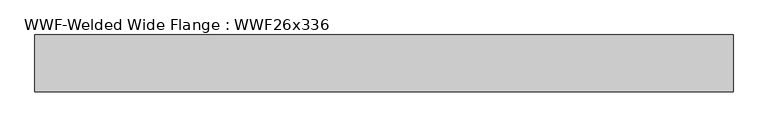
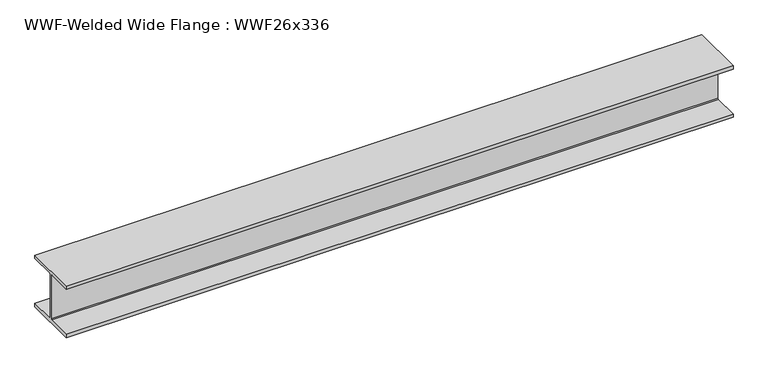
"""IFC4 building model written with IfcOpenShell, lengths in millimetres: beam geometry, WWF-Welded Wide Flange : WWF26x336."""

from ifc_helpers import new_model, si_unit, frame, origin, place, context, project, spatial, polyline, outline, extrude, source, transform, mapped, element, save


def wwf_welded_wide_flange_wwf26x336_71f8c54e(model_context):
    return source(origin(), model_context, "Body", "SweptSolid", [
        extrude(outline(polyline([(324.993, -284.988), (324.993, -324.993), (-324.993, -324.993), (-324.993, -284.988), (-20.6375, -284.988), (-9.9949, -274.3454), (-9.9949, 274.3454), (-20.6375, 284.988), (-324.993, 284.988), (-324.993, 324.993), (324.993, 324.993), (324.993, 284.988), (20.6375, 284.988), (9.9949, 274.3454), (9.9949, -274.3454), (20.6375, -284.988), (324.993, -284.988)])), frame((-3934.8877112, 0.0, 0.0), z_axis=(1.0, 0.0, 0.0), x_axis=(0.0, 1.0, 0.0)), (0.0, 0.0, 1.0), 7999.1183534),
    ])


if __name__ == "__main__":
    model = new_model("IFC4")
    model_context = context("Model", 3, world=origin())
    ifc_project = project(units=[si_unit("LENGTHUNIT", "METRE", prefix="MILLI")], contexts=[model_context])
    site = spatial("IfcSite", under=ifc_project)
    building = spatial("IfcBuilding", under=site)
    placement = place(None, origin())
    wwf_welded_wide_flange_wwf26x336_shape = wwf_welded_wide_flange_wwf26x336_71f8c54e(model_context)
    element("IfcBeam", 1, ObjectType="WWF-Welded Wide Flange : WWF26x336", at=placement, inside=building, context=model_context, shape_type="MappedRepresentation", body=[
        mapped(wwf_welded_wide_flange_wwf26x336_shape, transform((0.0, 0.0, 0.0), x_axis=(1.0, 0.0, 0.0), y_axis=(0.0, 1.0, 0.0), z_axis=(0.0, 0.0, 1.0))),
    ])
    save(model, "model.ifc")

# Revit data of these elements
# Type "WWF-Welded Wide Flange : WWF26x336"
#   Assembly Code = "B10"
#   Nominal d = "12"
#   W = 336
#   Length [instance default] = 1524 mm
#   bf = 649.986 mm
#   d = 649.986 mm
#   k = 20.638 mm
#   tf = 40.005 mm
#   tw = 19.99 mm
#   A = 0.0635483 m²
#   Structural Material [instance default] = Steel ASTM A572
# Element 1 (IfcBeam, "WWF-Welded Wide Flange : WWF26x336")
#   Structural Material = Metal - Steel 43-275
#   Materials on its faces: "Metal - Steel 43-275"
# Materials
#   "Steel ASTM A572": class "Metal", colour RGB 247 247 247, transparency 0, Description = "Structural steel, high strength low alloy, ASTM - A572 - 50", Cost = 0
#   "Metal - Steel 43-275": class "Metal", colour RGB 247 247 247, transparency 0, Cost = 0
